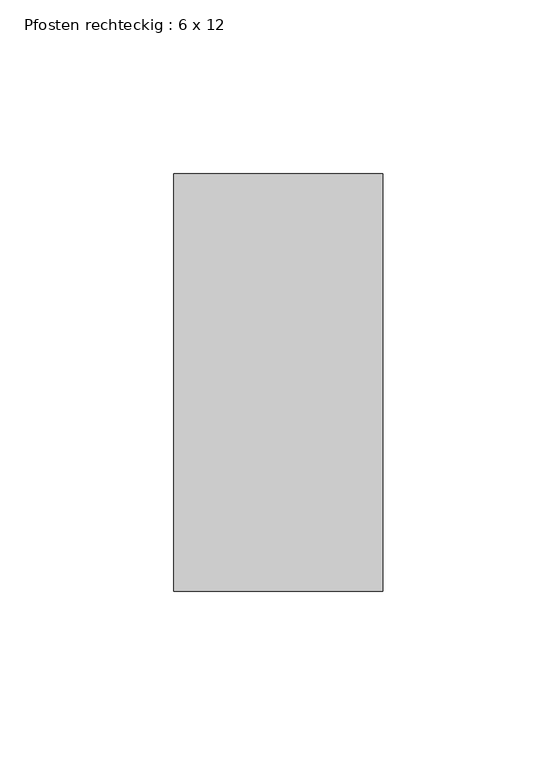
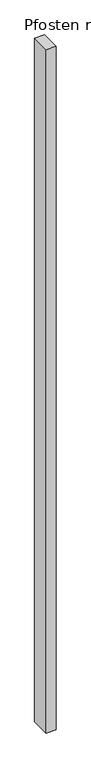
"""IFC4 building model written with IfcOpenShell, lengths in millimetres: member geometry, Pfosten rechteckig : 6 x 12."""

from ifc_helpers import new_model, si_unit, frame, origin, place, context, project, spatial, polyline, outline, extrude, source, transform, mapped, element, save


def pfosten_rechteckig_6_x_12_3c96996c(model_context):
    return source(origin(), model_context, "Body", "SweptSolid", [
        extrude(outline(polyline([(0.0, 60.0), (0.0, -60.0), (-60.0, -60.0), (-60.0, 60.0), (0.0, 60.0)])), frame((0.0, 0.0, -4356.6788019), z_axis=(0.0, 0.0, 1.0), x_axis=(1.0, 0.0, 0.0)), (0.0, 0.0, 1.0), 4356.6788019),
    ])


if __name__ == "__main__":
    model = new_model("IFC4")
    model_context = context("Model", 3, world=origin())
    ifc_project = project(units=[si_unit("LENGTHUNIT", "METRE", prefix="MILLI")], contexts=[model_context])
    site = spatial("IfcSite", under=ifc_project)
    building = spatial("IfcBuilding", under=site)
    placement = place(None, origin())
    pfosten_rechteckig_6_x_12_shape = pfosten_rechteckig_6_x_12_3c96996c(model_context)
    element("IfcMember", 1, ObjectType="Pfosten rechteckig : 6 x 12", at=placement, inside=building, context=model_context, shape_type="MappedRepresentation", body=[
        mapped(pfosten_rechteckig_6_x_12_shape, transform((0.0, 0.0, 0.0), x_axis=(1.0, 0.0, 0.0), y_axis=(0.0, 1.0, 0.0), z_axis=(0.0, 0.0, 1.0))),
    ])
    save(model, "model.ifc")

# Revit data of these elements
# Type "Pfosten rechteckig : 6 x 12"
#   built-in parameter 1007304 = 0.393701 (stored number, unit not read)
#   built-in parameter 1007301 = 0.0984252 (stored number, unit not read)
#   built-in parameter 1007300 = 0.0984252 (stored number, unit not read)
# Element 1 (IfcMember, "Pfosten rechteckig : 6 x 12")
#   Materials on its faces: "Metall - verzinkt"
# Materials
#   "Metall - verzinkt": class "Allgemeines", colour RGB 200 200 200, transparency 0, Cost = 0
